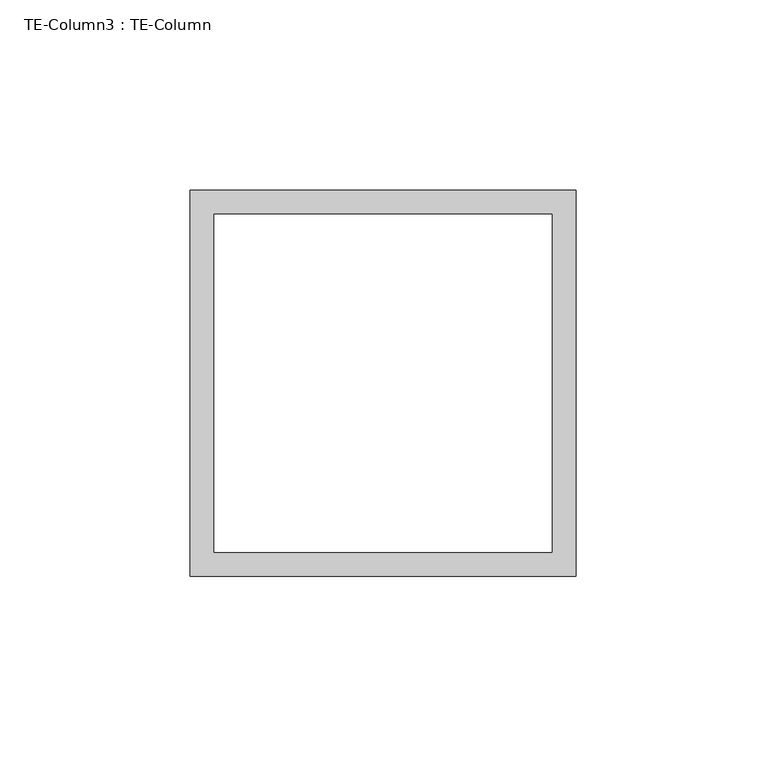
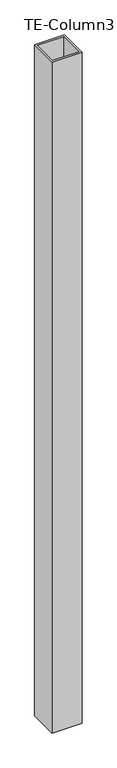
"""IFC4 building model written with IfcOpenShell, lengths in millimetres: proxy geometry, TE-Column3 : TE-Column."""

from ifc_helpers import new_model, si_unit, frame, origin, place, context, project, spatial, polyline, outline, extrude, source, transform, mapped, element, save


def te_column3_te_column_f065ebbf(model_context):
    return source(origin(), model_context, "Body", "SweptSolid", [
        extrude(outline(polyline([(590318.6434739, -532931.4413841), (590217.0434739, -532931.4413841), (590217.0434739, -532829.8413841), (590318.6434739, -532829.8413841), (590318.6434739, -532931.4413841)]), holes=[polyline([(590312.2934739, -532836.1913841), (590223.3934739, -532836.1913841), (590223.3934739, -532925.0913841), (590312.2934739, -532925.0913841), (590312.2934739, -532836.1913841)])]), frame((0.0, 0.0, 28.575), z_axis=(0.0, 0.0, 1.0), x_axis=(1.0, 0.0, 0.0)), (0.0, 0.0, 1.0), 2406.65),
    ])


if __name__ == "__main__":
    model = new_model("IFC4")
    model_context = context("Model", 3, world=origin())
    ifc_project = project(units=[si_unit("LENGTHUNIT", "METRE", prefix="MILLI")], contexts=[model_context])
    site = spatial("IfcSite", under=ifc_project)
    building = spatial("IfcBuilding", under=site)
    placement = place(None, origin())
    te_column3_te_column_shape = te_column3_te_column_f065ebbf(model_context)
    element("IfcBuildingElementProxy", 1, Name="TE-Column3 : TE-Column", ObjectType="TE-Column3 : TE-Column", at=placement, inside=building, context=model_context, shape_type="MappedRepresentation", body=[
        mapped(te_column3_te_column_shape, transform((0.0, 0.0, 0.0), x_axis=(1.0, 0.0, 0.0), y_axis=(0.0, 1.0, 0.0), z_axis=(0.0, 0.0, 1.0))),
    ])
    save(model, "model.ifc")

# Revit data of these elements
# Element 1 (IfcBuildingElementProxy, "TE-Column3 : TE-Column")
#   Materials on its faces: "4\"X4\" GALV. HSS TUBING"
# Materials
#   "4\"X4\" GALV. HSS TUBING": class "Generic", colour RGB 211 211 207, transparency 0, Cost = 0
